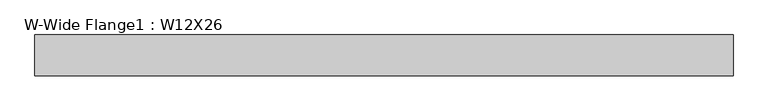
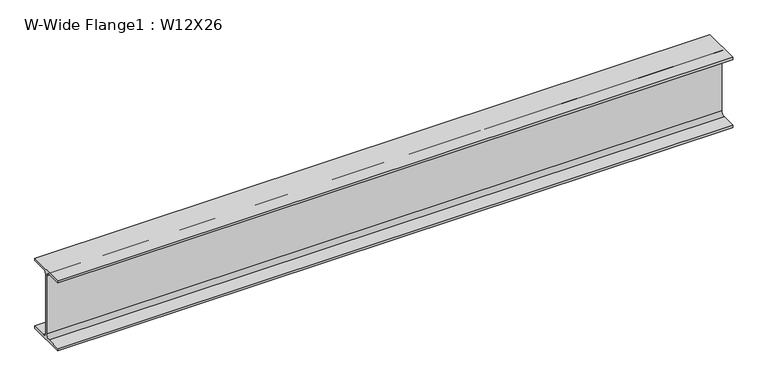
"""IFC4 building model written with IfcOpenShell, lengths in millimetres: beam geometry, W-Wide Flange1 : W12X26."""

from ifc_helpers import new_model, si_unit, point, frame, frame_2d, origin, place, context, project, spatial, polyline, circle_curve, trimmed, segment, composite_curve, outline, extrude, source, transform, mapped, element, save


def w_wide_flange1_w12x26_50a0faab(model_context):
    return source(origin(), model_context, "Body", "SweptSolid", [
        extrude(outline(composite_curve([segment(polyline([(82.423, -145.288), (82.423, -154.94), (-82.423, -154.94), (-82.423, -145.288), (-20.2565, -145.288)]), True, "CONTINUOUS"), segment(trimmed(circle_curve(frame_2d((-20.2565, -127.9525)), 17.3355), [point((-20.2565, -145.288))], [point((-2.921, -127.9525))], True, "CARTESIAN"), True, "CONTINUOUS"), segment(polyline([(-2.921, -127.9525), (-2.921, 127.9525)]), True, "CONTINUOUS"), segment(trimmed(circle_curve(frame_2d((-20.2565, 127.9525)), 17.3355), [point((-2.921, 127.9525))], [point((-20.2565, 145.288))], True, "CARTESIAN"), True, "CONTINUOUS"), segment(polyline([(-20.2565, 145.288), (-82.423, 145.288), (-82.423, 154.94), (82.423, 154.94), (82.423, 145.288), (20.2565, 145.288)]), True, "CONTINUOUS"), segment(trimmed(circle_curve(frame_2d((20.2565, 127.9525)), 17.3355), [point((20.2565, 145.288))], [point((2.921, 127.9525))], True, "CARTESIAN"), True, "CONTINUOUS"), segment(polyline([(2.921, 127.9525), (2.921, -127.9525)]), True, "CONTINUOUS"), segment(trimmed(circle_curve(frame_2d((20.2565, -127.9525)), 17.3355), [point((2.921, -127.9525))], [point((20.2565, -145.288))], True, "CARTESIAN"), True, "CONTINUOUS"), segment(polyline([(20.2565, -145.288), (82.423, -145.288)]), True, "CONTINUOUS")], self_intersect=False)), frame((-1358.9827624, 0.0, 0.0), z_axis=(1.0, 0.0, 0.0), x_axis=(0.0, 1.0, 0.0)), (0.0, 0.0, 1.0), 2827.6581169),
    ])


if __name__ == "__main__":
    model = new_model("IFC4")
    model_context = context("Model", 3, world=origin())
    ifc_project = project(units=[si_unit("LENGTHUNIT", "METRE", prefix="MILLI")], contexts=[model_context])
    site = spatial("IfcSite", under=ifc_project)
    building = spatial("IfcBuilding", under=site)
    placement = place(None, origin())
    w_wide_flange1_w12x26_shape = w_wide_flange1_w12x26_50a0faab(model_context)
    element("IfcBeam", 1, ObjectType="W-Wide Flange1 : W12X26", at=placement, inside=building, context=model_context, shape_type="MappedRepresentation", body=[
        mapped(w_wide_flange1_w12x26_shape, transform((0.0, 0.0, 0.0), x_axis=(1.0, 0.0, 0.0), y_axis=(0.0, 1.0, 0.0), z_axis=(0.0, 0.0, 1.0))),
    ])
    save(model, "model.ifc")

# Revit data of these elements
# Type "W-Wide Flange1 : W12X26"
#   Assembly Code = "B10"
#   W = 26
#   Start Extension Calculation [instance default] = 10' - 0"
#   Start Extension [instance default] = -0' - 0 1/2"
#   End Extension Calculation [instance default] = 10' - 0"
#   End Extension [instance default] = -0' - 0 1/2"
#   Length [instance default] = 5' - 0"
#   bf = 0' - 6.49"
#   d = 1' - 0.2"
#   k = 0' - 1 1/16"
#   k2 = 0' - 0.6825"
#   tf = 0' - 0.38"
#   tw = 0' - 0.23"
#   A = 0.053125 SF
#   Structural Material [instance default] = Metal - Steel - ASTM A992
# Element 1 (IfcBeam, "W-Wide Flange1 : W12X26")
#   Materials on its faces: "Metal - Steel - ASTM A992"
# Materials
#   "Metal - Steel - ASTM A992": class "Metal", colour RGB 199 199 199, transparency 0
